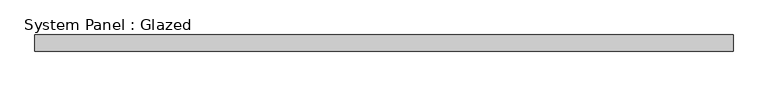
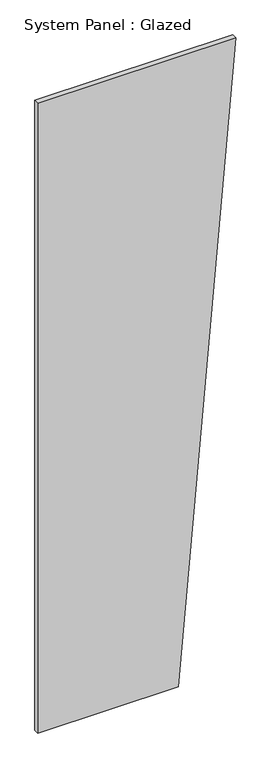
"""IFC4 building model written with IfcOpenShell, lengths in millimetres: plate geometry, System Panel : Glazed."""

from ifc_helpers import new_model, si_unit, frame, origin, place, context, project, spatial, polyline, outline, extrude, source, transform, mapped, element, save


def system_panel_glazed_127879aa(model_context):
    return source(origin(), model_context, "Body", "SweptSolid", [
        extrude(outline(polyline([(0.0, -543.7370389), (0.0, 228.6), (3657.6, 543.7370389), (3657.6, -543.7370389), (0.0, -543.7370389)])), frame((0.0, -44.45, 0.0), z_axis=(0.0, 1.0, 0.0), x_axis=(0.0, 0.0, 1.0)), (0.0, 0.0, 1.0), 25.4),
    ])


if __name__ == "__main__":
    model = new_model("IFC4")
    model_context = context("Model", 3, world=origin())
    ifc_project = project(units=[si_unit("LENGTHUNIT", "METRE", prefix="MILLI")], contexts=[model_context])
    site = spatial("IfcSite", under=ifc_project)
    building = spatial("IfcBuilding", under=site)
    placement = place(None, origin())
    system_panel_glazed_shape = system_panel_glazed_127879aa(model_context)
    element("IfcPlate", 1, ObjectType="System Panel : Glazed", at=placement, inside=building, context=model_context, shape_type="MappedRepresentation", body=[
        mapped(system_panel_glazed_shape, transform((0.0, 0.0, 0.0), x_axis=(1.0, 0.0, 0.0), y_axis=(0.0, 1.0, 0.0), z_axis=(0.0, 0.0, 1.0))),
    ])
    save(model, "model.ifc")

# Revit data of these elements
# Type "System Panel : Glazed"
#   Construction Type Id = "GSP4R"
#   Analytic Construction = "1/8 in Pilkington single glazing"
#   Visual Light Transmittance = 0.9
#   Solar Heat Gain Coefficient = 0.86
#   Heat Transfer Coefficient (U) = 1.18115 BTU/(h·ft²·°F)
#   Define Thermal Properties by = 1
# Element 1 (IfcPlate, "System Panel : Glazed")
#   Materials on its faces: "Glass"
# Materials
#   "Glass": class "Glass", colour RGB 0 128 192, transparency 0.75, Description = "Soda Lime Glass", Cost = 0
